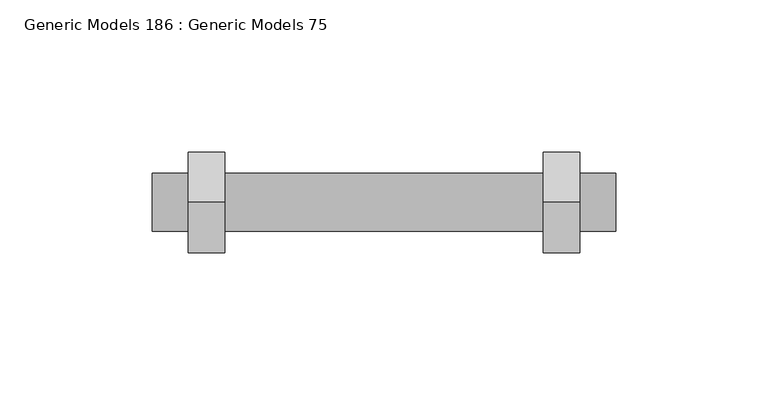
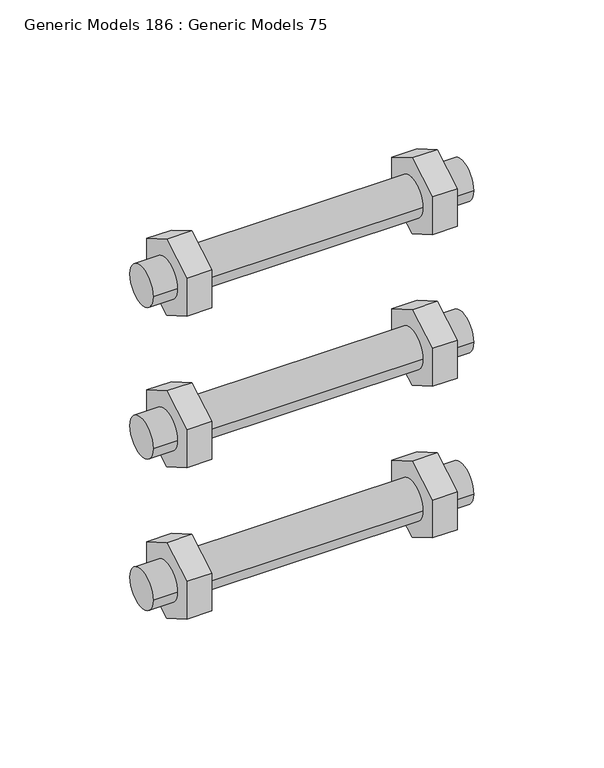
"""IFC4 building model written with IfcOpenShell, lengths in millimetres: proxy geometry, Generic Models 186 : Generic Models 75."""

import ifcopenshell
import ifcopenshell.guid

model = None  # the IFC model being written
_history = None  # IfcOwnerHistory: only IFC2X3 demands one
_inside = {}  # id of a spatial element -> (the spatial element, [elements in it])
_under = {}  # id of a project, library or spatial element -> (it, [spatial elements below it])
_declared = {}  # id of a project -> (the project, [libraries it declares])
_typed = {}  # id of a type object -> (the type object, [elements of that type])
_made_of = {}  # id of a material, layer set ... -> (it, [elements and type objects made of it])


def new_model(schema):
    """Start an empty IFC model of exactly this schema.

    Asked for "IFC4X3", IfcOpenShell would pick the latest addendum, in which some entities
    have other attributes; the version numbers below select the first issue.
    IFC2X3 requires an IfcOwnerHistory on every rooted entity: one is made here for all.
    """
    global model, _history
    if schema == "IFC4X3":
        model = ifcopenshell.file(schema_version=(4, 3, 0, 0))
    else:
        model = ifcopenshell.file(schema=schema)
    _inside.clear()
    _under.clear()
    _declared.clear()
    _typed.clear()
    _made_of.clear()
    _history = None
    if model.schema == "IFC2X3":
        org = make("IfcOrganization", Name="unknown")
        user = make(
            "IfcPersonAndOrganization",
            ThePerson=make("IfcPerson", FamilyName="unknown"),
            TheOrganization=org,
        )
        app = make(
            "IfcApplication",
            ApplicationDeveloper=org,
            Version="unknown",
            ApplicationFullName="unknown",
            ApplicationIdentifier="unknown",
        )
        _history = make(
            "IfcOwnerHistory",
            OwningUser=user,
            OwningApplication=app,
            ChangeAction="ADDED",
            CreationDate=0,
        )
    return model


def make(cls, **values):
    """One entity of the class cls with the attributes given. An attribute that is None is left unset."""
    return model.create_entity(
        cls, **{name: value for name, value in values.items() if value is not None}
    )


def rooted(cls, **values):
    """An entity with a GlobalId (a new one), such as an element, a storey or a relation."""
    return make(cls, GlobalId=ifcopenshell.guid.new(), OwnerHistory=_history, **values)


def si_unit(unit_type, name, prefix=None):
    """IfcSIUnit, for example si_unit("LENGTHUNIT", "METRE", prefix="MILLI")."""
    return make("IfcSIUnit", UnitType=unit_type, Prefix=prefix, Name=name)


def assignment(units):
    """IfcUnitAssignment: the units of a project."""
    return None if units is None else make("IfcUnitAssignment", Units=units)


def point(xyz):
    """IfcCartesianPoint."""
    return None if xyz is None else make("IfcCartesianPoint", Coordinates=xyz)


def direction(xyz):
    """IfcDirection."""
    return None if xyz is None else make("IfcDirection", DirectionRatios=xyz)


def frame(location, z_axis=None, x_axis=None):
    """IfcAxis2Placement3D, a coordinate frame: its origin and axes. An axis left out is left unset."""
    return make(
        "IfcAxis2Placement3D",
        Location=point(location),
        Axis=direction(z_axis),
        RefDirection=direction(x_axis),
    )


def frame_2d(location, x_axis=None):
    """IfcAxis2Placement2D, a coordinate frame in the plane: its origin and x axis."""
    return make(
        "IfcAxis2Placement2D", Location=point(location), RefDirection=direction(x_axis)
    )


def origin():
    """The frame at (0, 0, 0) with its axes left unset."""
    return frame((0.0, 0.0, 0.0))


def place(relative_to, where):
    """IfcLocalPlacement: puts the frame where relative to a parent placement (None: the world)."""
    return make(
        "IfcLocalPlacement", PlacementRelTo=relative_to, RelativePlacement=where
    )


def context(
    kind, dimensions, precision=None, world=None, true_north=None, identifier=None
):
    """IfcGeometricRepresentationContext, for example the 3D "Model" context."""
    return make(
        "IfcGeometricRepresentationContext",
        ContextIdentifier=identifier,
        ContextType=kind,
        CoordinateSpaceDimension=dimensions,
        Precision=precision,
        WorldCoordinateSystem=world,
        TrueNorth=true_north,
    )


def project(units=None, contexts=None):
    """IfcProject with its units and contexts."""
    return rooted(
        "IfcProject",
        Name="project",
        RepresentationContexts=contexts,
        UnitsInContext=assignment(units),
    )


def spatial(cls, under=None, at=None, **own):
    """A site, building, storey or space (cls), placed at a placement, below another one or the project."""
    s = rooted(cls, ObjectPlacement=at, **own)
    if under is not None:
        _under.setdefault(under.id(), (under, []))[1].append(s)
    return s


def polyline(points):
    """IfcPolyline through the points."""
    return make("IfcPolyline", Points=[point(p) for p in points])


def circle_curve(where, radius):
    """IfcCircle in the frame where."""
    return make("IfcCircle", Position=where, Radius=radius)


def trimmed(basis, trim1, trim2, sense, master):
    """IfcTrimmedCurve: the piece of a basis curve between two trims."""
    return make(
        "IfcTrimmedCurve",
        BasisCurve=basis,
        Trim1=trim1,
        Trim2=trim2,
        SenseAgreement=sense,
        MasterRepresentation=master,
    )


def segment(curve, same_sense, transition):
    """IfcCompositeCurveSegment."""
    return make(
        "IfcCompositeCurveSegment",
        Transition=transition,
        SameSense=same_sense,
        ParentCurve=curve,
    )


def composite_curve(segments, self_intersect=None):
    """IfcCompositeCurve: segments joined end to end."""
    return make("IfcCompositeCurve", Segments=segments, SelfIntersect=self_intersect)


def outline(outer, holes=None, kind="AREA"):
    """IfcArbitraryClosedProfileDef: a profile drawn as a closed curve; with holes, ...WithVoids."""
    if holes is None:
        return make("IfcArbitraryClosedProfileDef", ProfileType=kind, OuterCurve=outer)
    return make(
        "IfcArbitraryProfileDefWithVoids",
        ProfileType=kind,
        OuterCurve=outer,
        InnerCurves=holes,
    )


def extrude(swept, where, along, depth):
    """IfcExtrudedAreaSolid: the profile swept, set in the frame where, extruded along a direction by depth."""
    return make(
        "IfcExtrudedAreaSolid",
        SweptArea=swept,
        Position=where,
        ExtrudedDirection=direction(along),
        Depth=depth,
    )


def shape(context_of_items, identifier, shape_type, items):
    """IfcShapeRepresentation: the items that make up one representation, for example the "Body"."""
    return make(
        "IfcShapeRepresentation",
        ContextOfItems=context_of_items,
        RepresentationIdentifier=identifier,
        RepresentationType=shape_type,
        Items=items,
    )


def source(mapping_origin, context_of_items, identifier, shape_type, items):
    """IfcRepresentationMap: a shape defined once, which mapped items show again and again."""
    return make(
        "IfcRepresentationMap",
        MappingOrigin=mapping_origin,
        MappedRepresentation=shape(context_of_items, identifier, shape_type, items),
    )


def transform(
    local_origin,
    x_axis=None,
    y_axis=None,
    z_axis=None,
    scale=None,
    scale2=None,
    scale3=None,
    uniform=True,
):
    """IfcCartesianTransformationOperator3D, or its non-uniform kind. x_axis, y_axis, z_axis: its Axis1, 2, 3."""
    if uniform:
        return make(
            "IfcCartesianTransformationOperator3D",
            Axis1=direction(x_axis),
            Axis2=direction(y_axis),
            LocalOrigin=point(local_origin),
            Scale=scale,
            Axis3=direction(z_axis),
        )
    return make(
        "IfcCartesianTransformationOperator3DnonUniform",
        Axis1=direction(x_axis),
        Axis2=direction(y_axis),
        LocalOrigin=point(local_origin),
        Scale=scale,
        Axis3=direction(z_axis),
        Scale2=scale2,
        Scale3=scale3,
    )


def mapped(mapping_source, mapping_target):
    """IfcMappedItem: shows the shape of a source again, moved by a transform."""
    return make(
        "IfcMappedItem", MappingSource=mapping_source, MappingTarget=mapping_target
    )


def made_of(thing, what):
    """Note that an element or type object is made of a material, layer set ...; save() writes the relation."""
    if what is not None:
        _made_of.setdefault(what.id(), (what, []))[1].append(thing)
    return thing


def element(
    cls,
    number,
    at=None,
    inside=None,
    cuts=None,
    type_object=None,
    material=None,
    context=None,
    identifier="Body",
    shape_type=None,
    held_by="IfcProductDefinitionShape",
    body=None,
    shapes=None,
    **own,
):
    """One element of the class cls, such as IfcWall. Its Tag is "e" and its number.

    at: its placement. inside: the storey or other place that contains it. cuts: it is an
    opening in that element (IfcRelVoidsElement). A single representation is given by context,
    identifier, shape_type and body (its items); several are given by shapes. held_by: the class
    of the entity that holds the representations. save() writes the other relations.
    """
    e = rooted(cls, Tag="e%d" % number, ObjectPlacement=at, **own)
    if body is not None:
        shapes = [shape(context, identifier, shape_type, body)]
    if shapes is not None:
        e.Representation = make(held_by, Representations=shapes)
    if inside is not None:
        _inside.setdefault(inside.id(), (inside, []))[1].append(e)
    if cuts is not None:
        rooted(
            "IfcRelVoidsElement", RelatingBuildingElement=cuts, RelatedOpeningElement=e
        )
    if type_object is not None:
        _typed.setdefault(type_object.id(), (type_object, []))[1].append(e)
    return made_of(e, material)


def aggregate(whole, parts):
    """IfcRelAggregates: a whole, such as a stair, and the parts it consists of."""
    return rooted("IfcRelAggregates", RelatingObject=whole, RelatedObjects=parts)


def save(model, path):
    """Write the relations noted so far, then the file.

    IfcRelAggregates (storeys below a building ...), IfcRelContainedInSpatialStructure (elements
    in a storey), IfcRelDefinesByType, IfcRelAssociatesMaterial and IfcRelDeclares: one each for
    every whole, place, type object, material and project.
    """
    for whole, parts in _under.values():
        aggregate(whole, parts)
    for where, things in _inside.values():
        rooted(
            "IfcRelContainedInSpatialStructure",
            RelatedElements=things,
            RelatingStructure=where,
        )
    for kind, things in _typed.values():
        rooted("IfcRelDefinesByType", RelatedObjects=things, RelatingType=kind)
    for what, things in _made_of.values():
        rooted("IfcRelAssociatesMaterial", RelatedObjects=things, RelatingMaterial=what)
    for by, libraries in _declared.values():
        rooted("IfcRelDeclares", RelatingContext=by, RelatedDefinitions=libraries)
    model.write(path)


def generic_models_186_generic_models_75_581a1899(model_context):
    return source(origin(), model_context, "Body", "SweptSolid", [
        extrude(outline(polyline([(36545.7042603, 269062.859622), (36562.2020442, 269072.384622), (36578.6998281, 269062.859622), (36578.6998281, 269043.809622), (36562.2020442, 269034.284622), (36545.7042603, 269043.809622), (36545.7042603, 269062.859622)])), frame((31918.2596032, 0.0, 0.0), z_axis=(1.0, 0.0, 0.0), x_axis=(0.0, 1.0, 0.0)), (0.0, 0.0, 1.0), 11.90625),
        extrude(outline(polyline([(36545.7042603, 268986.659622), (36562.2020442, 268996.184622), (36578.6998281, 268986.659622), (36578.6998281, 268967.609622), (36562.2020442, 268958.084622), (36545.7042603, 268967.609622), (36545.7042603, 268986.659622)])), frame((31918.2596032, 0.0, 0.0), z_axis=(1.0, 0.0, 0.0), x_axis=(0.0, 1.0, 0.0)), (0.0, 0.0, 1.0), 11.90625),
        extrude(outline(polyline([(36545.7042603, 268910.459622), (36562.2020442, 268919.984622), (36578.6998281, 268910.459622), (36578.6998281, 268891.409622), (36562.2020442, 268881.884622), (36545.7042603, 268891.409622), (36545.7042603, 268910.459622)])), frame((31918.2596032, 0.0, 0.0), z_axis=(1.0, 0.0, 0.0), x_axis=(0.0, 1.0, 0.0)), (0.0, 0.0, 1.0), 11.90625),
        extrude(outline(polyline([(36545.7042603, 269062.859622), (36562.2020442, 269072.384622), (36578.6998281, 269062.859622), (36578.6998281, 269043.809622), (36562.2020442, 269034.284622), (36545.7042603, 269043.809622), (36545.7042603, 269062.859622)])), frame((31801.5783532, 0.0, 0.0), z_axis=(1.0, 0.0, 0.0), x_axis=(0.0, 1.0, 0.0)), (0.0, 0.0, 1.0), 11.90625),
        extrude(outline(polyline([(36545.7042603, 268986.659622), (36562.2020442, 268996.184622), (36578.6998281, 268986.659622), (36578.6998281, 268967.609622), (36562.2020442, 268958.084622), (36545.7042603, 268967.609622), (36545.7042603, 268986.659622)])), frame((31801.5783532, 0.0, 0.0), z_axis=(1.0, 0.0, 0.0), x_axis=(0.0, 1.0, 0.0)), (0.0, 0.0, 1.0), 11.90625),
        extrude(outline(polyline([(36545.7042603, 268910.459622), (36562.2020442, 268919.984622), (36578.6998281, 268910.459622), (36578.6998281, 268891.409622), (36562.2020442, 268881.884622), (36545.7042603, 268891.409622), (36545.7042603, 268910.459622)])), frame((31801.5783532, 0.0, 0.0), z_axis=(1.0, 0.0, 0.0), x_axis=(0.0, 1.0, 0.0)), (0.0, 0.0, 1.0), 11.90625),
        extrude(outline(composite_curve([segment(trimmed(circle_curve(frame_2d((36562.2020442, 268977.134622)), 9.525), [point((36571.7270442, 268977.134622))], [point((36552.6770442, 268977.134622))], False, "CARTESIAN"), True, "CONTINUOUS"), segment(trimmed(circle_curve(frame_2d((36562.2020442, 268977.134622)), 9.525), [point((36552.6770442, 268977.134622))], [point((36571.7270442, 268977.134622))], False, "CARTESIAN"), True, "CONTINUOUS")], self_intersect=False)), frame((31789.6721032, 0.0, 0.0), z_axis=(1.0, 0.0, 0.0), x_axis=(0.0, 1.0, 0.0)), (0.0, 0.0, 1.0), 152.4),
        extrude(outline(composite_curve([segment(trimmed(circle_curve(frame_2d((36562.2020442, 268900.934622)), 9.525), [point((36571.7270442, 268900.934622))], [point((36552.6770442, 268900.934622))], False, "CARTESIAN"), True, "CONTINUOUS"), segment(trimmed(circle_curve(frame_2d((36562.2020442, 268900.934622)), 9.525), [point((36552.6770442, 268900.934622))], [point((36571.7270442, 268900.934622))], False, "CARTESIAN"), True, "CONTINUOUS")], self_intersect=False)), frame((31789.6721032, 0.0, 0.0), z_axis=(1.0, 0.0, 0.0), x_axis=(0.0, 1.0, 0.0)), (0.0, 0.0, 1.0), 152.4),
        extrude(outline(composite_curve([segment(trimmed(circle_curve(frame_2d((36562.2020442, 269053.334622)), 9.525), [point((36571.7270442, 269053.334622))], [point((36552.6770442, 269053.334622))], False, "CARTESIAN"), True, "CONTINUOUS"), segment(trimmed(circle_curve(frame_2d((36562.2020442, 269053.334622)), 9.525), [point((36552.6770442, 269053.334622))], [point((36571.7270442, 269053.334622))], False, "CARTESIAN"), True, "CONTINUOUS")], self_intersect=False)), frame((31789.6721032, 0.0, 0.0), z_axis=(1.0, 0.0, 0.0), x_axis=(0.0, 1.0, 0.0)), (0.0, 0.0, 1.0), 152.4),
    ])


if __name__ == "__main__":
    model = new_model("IFC4")
    model_context = context("Model", 3, world=origin())
    ifc_project = project(units=[si_unit("LENGTHUNIT", "METRE", prefix="MILLI")], contexts=[model_context])
    site = spatial("IfcSite", under=ifc_project)
    building = spatial("IfcBuilding", under=site)
    placement = place(None, origin())
    generic_models_186_generic_models_75_shape = generic_models_186_generic_models_75_581a1899(model_context)
    element("IfcBuildingElementProxy", 1, Name="Generic Models 186 : Generic Models 75", ObjectType="Generic Models 186 : Generic Models 75", at=placement, inside=building, context=model_context, shape_type="MappedRepresentation", body=[
        mapped(generic_models_186_generic_models_75_shape, transform((0.0, 0.0, 0.0), x_axis=(1.0, 0.0, 0.0), y_axis=(0.0, 1.0, 0.0), z_axis=(0.0, 0.0, 1.0))),
    ])
    save(model, "model.ifc")
